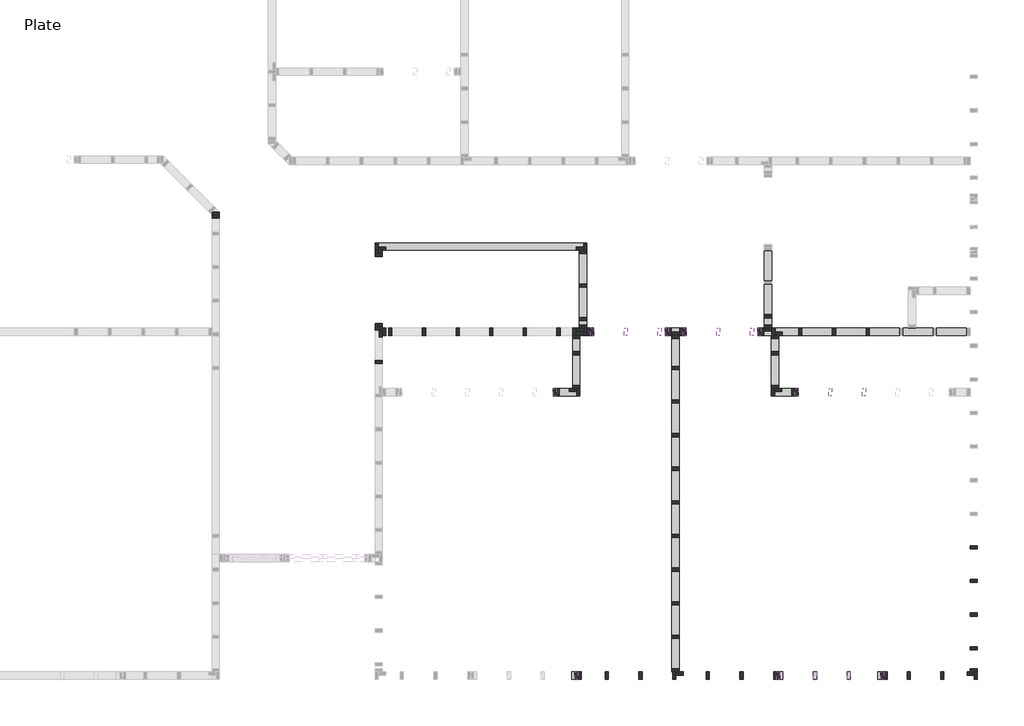
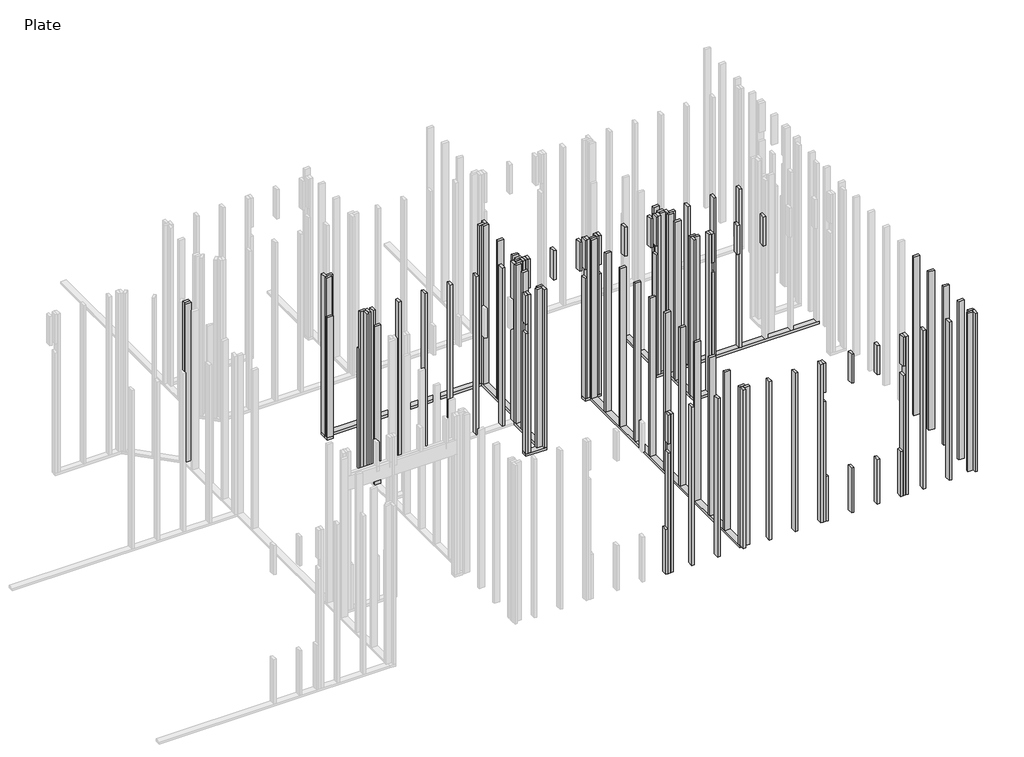
# One storey, part 2 of 5: 112 columns, 11 beams.
"""IFC4 building model written with IfcOpenShell, lengths in millimetres."""

import ifcopenshell
import ifcopenshell.guid

model = None  # the IFC model being written
_history = None  # IfcOwnerHistory: only IFC2X3 demands one
_inside = {}  # id of a spatial element -> (the spatial element, [elements in it])
_under = {}  # id of a project, library or spatial element -> (it, [spatial elements below it])
_declared = {}  # id of a project -> (the project, [libraries it declares])
_typed = {}  # id of a type object -> (the type object, [elements of that type])
_made_of = {}  # id of a material, layer set ... -> (it, [elements and type objects made of it])


def new_model(schema):
    """Start an empty IFC model of exactly this schema.

    Asked for "IFC4X3", IfcOpenShell would pick the latest addendum, in which some entities
    have other attributes; the version numbers below select the first issue.
    IFC2X3 requires an IfcOwnerHistory on every rooted entity: one is made here for all.
    """
    global model, _history
    if schema == "IFC4X3":
        model = ifcopenshell.file(schema_version=(4, 3, 0, 0))
    else:
        model = ifcopenshell.file(schema=schema)
    _inside.clear()
    _under.clear()
    _declared.clear()
    _typed.clear()
    _made_of.clear()
    _history = None
    if model.schema == "IFC2X3":
        org = make("IfcOrganization", Name="unknown")
        user = make(
            "IfcPersonAndOrganization",
            ThePerson=make("IfcPerson", FamilyName="unknown"),
            TheOrganization=org,
        )
        app = make(
            "IfcApplication",
            ApplicationDeveloper=org,
            Version="unknown",
            ApplicationFullName="unknown",
            ApplicationIdentifier="unknown",
        )
        _history = make(
            "IfcOwnerHistory",
            OwningUser=user,
            OwningApplication=app,
            ChangeAction="ADDED",
            CreationDate=0,
        )
    return model


def make(cls, **values):
    """One entity of the class cls with the attributes given. An attribute that is None is left unset."""
    return model.create_entity(
        cls, **{name: value for name, value in values.items() if value is not None}
    )


def rooted(cls, **values):
    """An entity with a GlobalId (a new one), such as an element, a storey or a relation."""
    return make(cls, GlobalId=ifcopenshell.guid.new(), OwnerHistory=_history, **values)


def si_unit(unit_type, name, prefix=None):
    """IfcSIUnit, for example si_unit("LENGTHUNIT", "METRE", prefix="MILLI")."""
    return make("IfcSIUnit", UnitType=unit_type, Prefix=prefix, Name=name)


def assignment(units):
    """IfcUnitAssignment: the units of a project."""
    return None if units is None else make("IfcUnitAssignment", Units=units)


def point(xyz):
    """IfcCartesianPoint."""
    return None if xyz is None else make("IfcCartesianPoint", Coordinates=xyz)


def direction(xyz):
    """IfcDirection."""
    return None if xyz is None else make("IfcDirection", DirectionRatios=xyz)


def frame(location, z_axis=None, x_axis=None):
    """IfcAxis2Placement3D, a coordinate frame: its origin and axes. An axis left out is left unset."""
    return make(
        "IfcAxis2Placement3D",
        Location=point(location),
        Axis=direction(z_axis),
        RefDirection=direction(x_axis),
    )


def origin():
    """The frame at (0, 0, 0) with its axes left unset."""
    return frame((0.0, 0.0, 0.0))


def place(relative_to, where):
    """IfcLocalPlacement: puts the frame where relative to a parent placement (None: the world)."""
    return make(
        "IfcLocalPlacement", PlacementRelTo=relative_to, RelativePlacement=where
    )


def context(
    kind, dimensions, precision=None, world=None, true_north=None, identifier=None
):
    """IfcGeometricRepresentationContext, for example the 3D "Model" context."""
    return make(
        "IfcGeometricRepresentationContext",
        ContextIdentifier=identifier,
        ContextType=kind,
        CoordinateSpaceDimension=dimensions,
        Precision=precision,
        WorldCoordinateSystem=world,
        TrueNorth=true_north,
    )


def project(units=None, contexts=None):
    """IfcProject with its units and contexts."""
    return rooted(
        "IfcProject",
        Name="project",
        RepresentationContexts=contexts,
        UnitsInContext=assignment(units),
    )


def spatial(cls, under=None, at=None, **own):
    """A site, building, storey or space (cls), placed at a placement, below another one or the project."""
    s = rooted(cls, ObjectPlacement=at, **own)
    if under is not None:
        _under.setdefault(under.id(), (under, []))[1].append(s)
    return s


def polyline(points):
    """IfcPolyline through the points."""
    return make("IfcPolyline", Points=[point(p) for p in points])


def outline(outer, holes=None, kind="AREA"):
    """IfcArbitraryClosedProfileDef: a profile drawn as a closed curve; with holes, ...WithVoids."""
    if holes is None:
        return make("IfcArbitraryClosedProfileDef", ProfileType=kind, OuterCurve=outer)
    return make(
        "IfcArbitraryProfileDefWithVoids",
        ProfileType=kind,
        OuterCurve=outer,
        InnerCurves=holes,
    )


def extrude(swept, where, along, depth):
    """IfcExtrudedAreaSolid: the profile swept, set in the frame where, extruded along a direction by depth."""
    return make(
        "IfcExtrudedAreaSolid",
        SweptArea=swept,
        Position=where,
        ExtrudedDirection=direction(along),
        Depth=depth,
    )


def shape(context_of_items, identifier, shape_type, items):
    """IfcShapeRepresentation: the items that make up one representation, for example the "Body"."""
    return make(
        "IfcShapeRepresentation",
        ContextOfItems=context_of_items,
        RepresentationIdentifier=identifier,
        RepresentationType=shape_type,
        Items=items,
    )


def source(mapping_origin, context_of_items, identifier, shape_type, items):
    """IfcRepresentationMap: a shape defined once, which mapped items show again and again."""
    return make(
        "IfcRepresentationMap",
        MappingOrigin=mapping_origin,
        MappedRepresentation=shape(context_of_items, identifier, shape_type, items),
    )


def transform(
    local_origin,
    x_axis=None,
    y_axis=None,
    z_axis=None,
    scale=None,
    scale2=None,
    scale3=None,
    uniform=True,
):
    """IfcCartesianTransformationOperator3D, or its non-uniform kind. x_axis, y_axis, z_axis: its Axis1, 2, 3."""
    if uniform:
        return make(
            "IfcCartesianTransformationOperator3D",
            Axis1=direction(x_axis),
            Axis2=direction(y_axis),
            LocalOrigin=point(local_origin),
            Scale=scale,
            Axis3=direction(z_axis),
        )
    return make(
        "IfcCartesianTransformationOperator3DnonUniform",
        Axis1=direction(x_axis),
        Axis2=direction(y_axis),
        LocalOrigin=point(local_origin),
        Scale=scale,
        Axis3=direction(z_axis),
        Scale2=scale2,
        Scale3=scale3,
    )


def mapped(mapping_source, mapping_target):
    """IfcMappedItem: shows the shape of a source again, moved by a transform."""
    return make(
        "IfcMappedItem", MappingSource=mapping_source, MappingTarget=mapping_target
    )


def made_of(thing, what):
    """Note that an element or type object is made of a material, layer set ...; save() writes the relation."""
    if what is not None:
        _made_of.setdefault(what.id(), (what, []))[1].append(thing)
    return thing


def element(
    cls,
    number,
    at=None,
    inside=None,
    cuts=None,
    type_object=None,
    material=None,
    context=None,
    identifier="Body",
    shape_type=None,
    held_by="IfcProductDefinitionShape",
    body=None,
    shapes=None,
    **own,
):
    """One element of the class cls, such as IfcWall. Its Tag is "e" and its number.

    at: its placement. inside: the storey or other place that contains it. cuts: it is an
    opening in that element (IfcRelVoidsElement). A single representation is given by context,
    identifier, shape_type and body (its items); several are given by shapes. held_by: the class
    of the entity that holds the representations. save() writes the other relations.
    """
    e = rooted(cls, Tag="e%d" % number, ObjectPlacement=at, **own)
    if body is not None:
        shapes = [shape(context, identifier, shape_type, body)]
    if shapes is not None:
        e.Representation = make(held_by, Representations=shapes)
    if inside is not None:
        _inside.setdefault(inside.id(), (inside, []))[1].append(e)
    if cuts is not None:
        rooted(
            "IfcRelVoidsElement", RelatingBuildingElement=cuts, RelatedOpeningElement=e
        )
    if type_object is not None:
        _typed.setdefault(type_object.id(), (type_object, []))[1].append(e)
    return made_of(e, material)


def aggregate(whole, parts):
    """IfcRelAggregates: a whole, such as a stair, and the parts it consists of."""
    return rooted("IfcRelAggregates", RelatingObject=whole, RelatedObjects=parts)


def save(model, path):
    """Write the relations noted so far, then the file.

    IfcRelAggregates (storeys below a building ...), IfcRelContainedInSpatialStructure (elements
    in a storey), IfcRelDefinesByType, IfcRelAssociatesMaterial and IfcRelDeclares: one each for
    every whole, place, type object, material and project.
    """
    for whole, parts in _under.values():
        aggregate(whole, parts)
    for where, things in _inside.values():
        rooted(
            "IfcRelContainedInSpatialStructure",
            RelatedElements=things,
            RelatingStructure=where,
        )
    for kind, things in _typed.values():
        rooted("IfcRelDefinesByType", RelatedObjects=things, RelatingType=kind)
    for what, things in _made_of.values():
        rooted("IfcRelAssociatesMaterial", RelatedObjects=things, RelatingMaterial=what)
    for by, libraries in _declared.values():
        rooted("IfcRelDeclares", RelatingContext=by, RelatedDefinitions=libraries)
    model.write(path)


def dimension_lumber_supporting_bottom_plate_c90501c4(model_context):
    return source(origin(), model_context, "Body", "SweptSolid", [
        extrude(outline(polyline([(1306.3140625, 44.45), (1306.3140625, -44.45), (-1261.8640625, -44.45), (-1261.8640625, 44.45), (1306.3140625, 44.45)])), frame((0.0, 0.0, -19.05), z_axis=(0.0, 0.0, 1.0), x_axis=(1.0, 0.0, 0.0)), (0.0, 0.0, 1.0), 38.1),
    ])


def dimension_lumber_supporting_bottom_plate_879a6a2b(model_context):
    return source(origin(), model_context, "Body", "SweptSolid", [
        extrude(outline(polyline([(2009.775, 44.45), (2009.775, -44.45), (-2060.575, -44.45), (-2060.575, 44.45), (2009.775, 44.45)])), frame((0.0, 0.0, -19.05), z_axis=(0.0, 0.0, 1.0), x_axis=(1.0, 0.0, 0.0)), (0.0, 0.0, 1.0), 38.1),
    ])


def dimension_lumber_supporting_bottom_plate_90e85d83(model_context):
    return source(origin(), model_context, "Body", "SweptSolid", [
        extrude(outline(polyline([(128.190625, 44.45), (128.190625, -44.45), (-128.190625, -44.45), (-128.190625, 44.45), (128.190625, 44.45)])), frame((0.0, 0.0, -19.05), z_axis=(0.0, 0.0, 1.0), x_axis=(1.0, 0.0, 0.0)), (0.0, 0.0, 1.0), 38.1),
    ])


def dimension_lumber_supporting_bottom_plate_7dbe58bc(model_context):
    return source(origin(), model_context, "Body", "SweptSolid", [
        extrude(outline(polyline([(469.9, 44.45), (469.9, -44.45), (-469.9, -44.45), (-469.9, 44.45), (469.9, 44.45)])), frame((0.0, 0.0, -19.05), z_axis=(0.0, 0.0, 1.0), x_axis=(1.0, 0.0, 0.0)), (0.0, 0.0, 1.0), 38.1),
    ])


def dimension_lumber_supporting_bottom_plate_050ef5e1(model_context):
    return source(origin(), model_context, "Body", "SweptSolid", [
        extrude(outline(polyline([(1279.525, 44.45), (1279.525, -44.45), (-1279.525, -44.45), (-1279.525, 44.45), (1279.525, 44.45)])), frame((0.0, 0.0, -19.05), z_axis=(0.0, 0.0, 1.0), x_axis=(1.0, 0.0, 0.0)), (0.0, 0.0, 1.0), 38.1),
    ])


def dimension_lumber_supporting_bottom_plate_723ed126(model_context):
    return source(origin(), model_context, "Body", "SweptSolid", [
        extrude(outline(polyline([(60.325, 44.45), (60.325, -44.45), (-15.875, -44.45), (-15.875, 44.45), (60.325, 44.45)])), frame((0.0, 0.0, -19.05), z_axis=(0.0, 0.0, 1.0), x_axis=(1.0, 0.0, 0.0)), (0.0, 0.0, 1.0), 38.1),
    ])


def dimension_lumber_supporting_bottom_plate_fcdf3739(model_context):
    return source(origin(), model_context, "Body", "SweptSolid", [
        extrude(outline(polyline([(352.425, 44.45), (352.425, -44.45), (-288.925, -44.45), (-288.925, 44.45), (352.425, 44.45)])), frame((0.0, 0.0, -19.05), z_axis=(0.0, 0.0, 1.0), x_axis=(1.0, 0.0, 0.0)), (0.0, 0.0, 1.0), 38.1),
    ])


def dimension_lumber_supporting_bottom_plate_c78b9630(model_context):
    return source(origin(), model_context, "Body", "SweptSolid", [
        extrude(outline(polyline([(488.95, 44.45), (488.95, -44.45), (-521.890625, -44.45), (-521.890625, 44.45), (488.95, 44.45)])), frame((0.0, 0.0, -19.05), z_axis=(0.0, 0.0, 1.0), x_axis=(1.0, 0.0, 0.0)), (0.0, 0.0, 1.0), 38.1),
    ])


def dimension_lumber_supporting_bottom_plate_50cface6(model_context):
    return source(origin(), model_context, "Body", "SweptSolid", [
        extrude(outline(polyline([(320.675, 44.45), (320.675, -44.45), (-320.675, -44.45), (-320.675, 44.45), (320.675, 44.45)])), frame((0.0, 0.0, -19.05), z_axis=(0.0, 0.0, 1.0), x_axis=(1.0, 0.0, 0.0)), (0.0, 0.0, 1.0), 38.1),
    ])


def dimension_lumber_supporting_bottom_plate_f7639587(model_context):
    return source(origin(), model_context, "Body", "SweptSolid", [
        extrude(outline(polyline([(184.9437503, 44.45), (184.9437503, -44.45), (-140.4937503, -44.45), (-140.4937503, 44.45), (184.9437503, 44.45)])), frame((0.0, 0.0, -19.05), z_axis=(0.0, 0.0, 1.0), x_axis=(1.0, 0.0, 0.0)), (0.0, 0.0, 1.0), 38.1),
    ])


def dimension_lumber_supporting_bottom_plate_f386abe9(model_context):
    return source(origin(), model_context, "Body", "SweptSolid", [
        extrude(outline(polyline([(184.15, 44.45), (184.15, -44.45), (-139.7, -44.45), (-139.7, 44.45), (184.15, 44.45)])), frame((0.0, 0.0, -19.05), z_axis=(0.0, 0.0, 1.0), x_axis=(1.0, 0.0, 0.0)), (0.0, 0.0, 1.0), 38.1),
    ])


def dimension_lumber_column_2x4_07183c39(model_context):
    return source(origin(), model_context, "Body", "SweptSolid", [
        extrude(outline(polyline([(19.05, 44.45), (19.05, -44.45), (-19.05, -44.45), (-19.05, 44.45), (19.05, 44.45)])), frame((0.0, 0.0, 56.35625), z_axis=(0.0, 0.0, 1.0), x_axis=(1.0, 0.0, 0.0)), (0.0, 0.0, 1.0), 2636.04375),
    ])


def dimension_lumber_column_2x4_f24b5bbb(model_context):
    return source(origin(), model_context, "Body", "SweptSolid", [
        extrude(outline(polyline([(19.05, -44.45), (-19.05, -44.45), (-19.05, 44.45), (19.05, 44.45), (19.05, -44.45)])), frame((0.0, 0.0, 56.35625), z_axis=(0.0, 0.0, 1.0), x_axis=(1.0, 0.0, 0.0)), (0.0, 0.0, 1.0), 2636.04375),
    ])


def dimension_lumber_column_2x4_0f816ddf(model_context):
    return source(origin(), model_context, "Body", "SweptSolid", [
        extrude(outline(polyline([(19.05, 44.45), (19.05, -44.45), (-19.05, -44.45), (-19.05, 44.45), (19.05, 44.45)])), frame((0.0, 0.0, 56.35625), z_axis=(0.0, 0.0, 1.0), x_axis=(1.0, 0.0, 0.0)), (0.0, 0.0, 1.0), 1999.853125),
    ])


def dimension_lumber_column_2x4_c2f848da(model_context):
    return source(origin(), model_context, "Body", "SweptSolid", [
        extrude(outline(polyline([(19.05, 44.45), (19.05, -44.45), (-19.05, -44.45), (-19.05, 44.45), (19.05, 44.45)])), frame((0.0, 0.0, 2208.609375), z_axis=(0.0, 0.0, 1.0), x_axis=(1.0, 0.0, 0.0)), (0.0, 0.0, 1.0), 483.790625),
    ])


def dimension_lumber_column_2x4_35883525(model_context):
    return source(origin(), model_context, "Body", "SweptSolid", [
        extrude(outline(polyline([(19.05, 44.45), (19.05, -44.45), (-19.05, -44.45), (-19.05, 44.45), (19.05, 44.45)])), frame((0.0, 0.0, 56.35625), z_axis=(0.0, 0.0, 1.0), x_axis=(1.0, 0.0, 0.0)), (0.0, 0.0, 1.0), 742.553125),
    ])


model = new_model("IFC4")

# Units and contexts
model_context = context("Model", 3, world=origin())
ifc_project = project(units=[si_unit("LENGTHUNIT", "METRE", prefix="MILLI")], contexts=[model_context])

# Site, building, storey
site = spatial("IfcSite", under=ifc_project)
building = spatial("IfcBuilding", under=site)
storey = spatial("IfcBuildingStorey", under=building, Name="Plate", Elevation=56.35625)

# Beams
placement = place(None, origin())
dimension_lumber_supporting_bottom_plate_shape = dimension_lumber_supporting_bottom_plate_c90501c4(model_context)
element("IfcBeam", 1, ObjectType="Dimension Lumber : Supporting Bottom Plate", at=placement, inside=storey, context=model_context, shape_type="MappedRepresentation", body=[
    mapped(dimension_lumber_supporting_bottom_plate_shape, transform((11893.3082124, -1545.8540947, 37.30625), x_axis=(-1.0, 0.0, 0.0), y_axis=(0.0, -1.0, 0.0), z_axis=(0.0, 0.0, 1.0))),
])
dimension_lumber_supporting_bottom_plate_2_shape = dimension_lumber_supporting_bottom_plate_879a6a2b(model_context)
element("IfcBeam", 2, ObjectType="Dimension Lumber : Supporting Bottom Plate", at=placement, inside=storey, context=model_context, shape_type="MappedRepresentation", body=[
    mapped(dimension_lumber_supporting_bottom_plate_2_shape, transform((9597.5847749, -3600.0790947, 37.30625), x_axis=(0.0, 1.0, 0.0), y_axis=(-1.0, 0.0, 0.0), z_axis=(0.0, 0.0, 1.0))),
])
dimension_lumber_supporting_bottom_plate_3_shape = dimension_lumber_supporting_bottom_plate_90e85d83(model_context)
element("IfcBeam", 3, ObjectType="Dimension Lumber : Supporting Bottom Plate", at=placement, inside=storey, context=model_context, shape_type="MappedRepresentation", body=[
    mapped(dimension_lumber_supporting_bottom_plate_3_shape, transform((9597.5847749, -1545.8540947, 37.30625), x_axis=(-1.0, 0.0, 0.0), y_axis=(0.0, -1.0, 0.0), z_axis=(0.0, 0.0, 1.0))),
])
dimension_lumber_supporting_bottom_plate_4_shape = dimension_lumber_supporting_bottom_plate_7dbe58bc(model_context)
element("IfcBeam", 4, ObjectType="Dimension Lumber : Supporting Bottom Plate", at=placement, inside=storey, context=model_context, shape_type="MappedRepresentation", body=[
    mapped(dimension_lumber_supporting_bottom_plate_4_shape, transform((8479.9847749, -1031.5040947, 37.30625), x_axis=(0.0, 1.0, 0.0), y_axis=(-1.0, 0.0, 0.0), z_axis=(0.0, 0.0, 1.0))),
])
dimension_lumber_supporting_bottom_plate_5_shape = dimension_lumber_supporting_bottom_plate_050ef5e1(model_context)
element("IfcBeam", 5, ObjectType="Dimension Lumber : Supporting Bottom Plate", at=placement, inside=storey, context=model_context, shape_type="MappedRepresentation", body=[
    mapped(dimension_lumber_supporting_bottom_plate_5_shape, transform((7244.9097749, -517.1540947, 37.30625), x_axis=(-1.0, 0.0, 0.0), y_axis=(0.0, -1.0, 0.0), z_axis=(0.0, 0.0, 1.0))),
])
dimension_lumber_supporting_bottom_plate_6_shape = dimension_lumber_supporting_bottom_plate_723ed126(model_context)
element("IfcBeam", 6, ObjectType="Dimension Lumber : Supporting Bottom Plate", at=placement, inside=storey, context=model_context, shape_type="MappedRepresentation", body=[
    mapped(dimension_lumber_supporting_bottom_plate_6_shape, transform((6009.8347749, -577.4790947, 37.30625), x_axis=(0.0, -1.0, 0.0), y_axis=(1.0, 0.0, 0.0), z_axis=(0.0, 0.0, 1.0))),
])
dimension_lumber_supporting_bottom_plate_7_shape = dimension_lumber_supporting_bottom_plate_fcdf3739(model_context)
element("IfcBeam", 7, ObjectType="Dimension Lumber : Supporting Bottom Plate", at=placement, inside=storey, context=model_context, shape_type="MappedRepresentation", body=[
    mapped(dimension_lumber_supporting_bottom_plate_7_shape, transform((8397.4347755, -1942.7290947, 37.30625), x_axis=(0.0, 1.0, 0.0), y_axis=(-1.0, 0.0, 0.0), z_axis=(0.0, 0.0, 1.0))),
])
dimension_lumber_supporting_bottom_plate_8_shape = dimension_lumber_supporting_bottom_plate_c78b9630(model_context)
element("IfcBeam", 8, ObjectType="Dimension Lumber : Supporting Bottom Plate", at=placement, inside=storey, context=model_context, shape_type="MappedRepresentation", body=[
    mapped(dimension_lumber_supporting_bottom_plate_8_shape, transform((10715.1847749, -1012.4540947, 37.30625), x_axis=(0.0, -1.0, 0.0), y_axis=(1.0, 0.0, 0.0), z_axis=(0.0, 0.0, 1.0))),
])
dimension_lumber_supporting_bottom_plate_9_shape = dimension_lumber_supporting_bottom_plate_50cface6(model_context)
element("IfcBeam", 9, ObjectType="Dimension Lumber : Supporting Bottom Plate", at=placement, inside=storey, context=model_context, shape_type="MappedRepresentation", body=[
    mapped(dimension_lumber_supporting_bottom_plate_9_shape, transform((10799.3222749, -1910.9790947, 37.30625), x_axis=(0.0, 1.0, 0.0), y_axis=(-1.0, 0.0, 0.0), z_axis=(0.0, 0.0, 1.0))),
])
dimension_lumber_supporting_bottom_plate_10_shape = dimension_lumber_supporting_bottom_plate_f7639587(model_context)
element("IfcBeam", 10, ObjectType="Dimension Lumber : Supporting Bottom Plate", at=placement, inside=storey, context=model_context, shape_type="MappedRepresentation", body=[
    mapped(dimension_lumber_supporting_bottom_plate_10_shape, transform((8256.9410252, -2276.1040947, 37.30625), x_axis=(1.0, 0.0, 0.0), y_axis=(0.0, 1.0, 0.0), z_axis=(0.0, 0.0, 1.0))),
])
dimension_lumber_supporting_bottom_plate_11_shape = dimension_lumber_supporting_bottom_plate_f386abe9(model_context)
element("IfcBeam", 11, ObjectType="Dimension Lumber : Supporting Bottom Plate", at=placement, inside=storey, context=model_context, shape_type="MappedRepresentation", body=[
    mapped(dimension_lumber_supporting_bottom_plate_11_shape, transform((10939.0222749, -2276.1040947, 37.30625), x_axis=(-1.0, 0.0, 0.0), y_axis=(0.0, -1.0, 0.0), z_axis=(0.0, 0.0, 1.0))),
])

# Columns
dimension_lumber_column_2x4_shape = dimension_lumber_column_2x4_07183c39(model_context)
element("IfcColumn", 12, ObjectType="Dimension Lumber-Column : 2x4", at=placement, inside=storey, context=model_context, shape_type="MappedRepresentation", body=[
    mapped(dimension_lumber_column_2x4_shape, transform((10799.3222749, -5705.1040947, 0.0), x_axis=(1.0, 0.0, 0.0), y_axis=(0.0, 1.0, 0.0), z_axis=(0.0, 0.0, 1.0))),
])
element("IfcColumn", 13, ObjectType="Dimension Lumber-Column : 2x4", at=placement, inside=storey, context=model_context, shape_type="MappedRepresentation", body=[
    mapped(dimension_lumber_column_2x4_shape, transform((10392.9222749, -5705.1040947, 0.0), x_axis=(1.0, 0.0, 0.0), y_axis=(0.0, 1.0, 0.0), z_axis=(0.0, 0.0, 1.0))),
])
element("IfcColumn", 14, ObjectType="Dimension Lumber-Column : 2x4", at=placement, inside=storey, context=model_context, shape_type="MappedRepresentation", body=[
    mapped(dimension_lumber_column_2x4_shape, transform((9986.5222749, -5705.1040947, 0.0), x_axis=(1.0, 0.0, 0.0), y_axis=(0.0, 1.0, 0.0), z_axis=(0.0, 0.0, 1.0))),
])
element("IfcColumn", 15, ObjectType="Dimension Lumber-Column : 2x4", at=placement, inside=storey, context=model_context, shape_type="MappedRepresentation", body=[
    mapped(dimension_lumber_column_2x4_shape, transform((9580.1222749, -5705.1040947, 0.0), x_axis=(1.0, 0.0, 0.0), y_axis=(0.0, 1.0, 0.0), z_axis=(0.0, 0.0, 1.0))),
])
element("IfcColumn", 16, ObjectType="Dimension Lumber-Column : 2x4", at=placement, inside=storey, context=model_context, shape_type="MappedRepresentation", body=[
    mapped(dimension_lumber_column_2x4_shape, transform((9173.7222749, -5705.1040947, 0.0), x_axis=(1.0, 0.0, 0.0), y_axis=(0.0, 1.0, 0.0), z_axis=(0.0, 0.0, 1.0))),
])
element("IfcColumn", 17, ObjectType="Dimension Lumber-Column : 2x4", at=placement, inside=storey, context=model_context, shape_type="MappedRepresentation", body=[
    mapped(dimension_lumber_column_2x4_shape, transform((8767.3222749, -5705.1040947, 0.0), x_axis=(1.0, 0.0, 0.0), y_axis=(0.0, 1.0, 0.0), z_axis=(0.0, 0.0, 1.0))),
])
element("IfcColumn", 18, ObjectType="Dimension Lumber-Column : 2x4", at=placement, inside=storey, context=model_context, shape_type="MappedRepresentation", body=[
    mapped(dimension_lumber_column_2x4_shape, transform((13199.6222749, -4154.1165947, 0.0), x_axis=(0.0, 1.0, 0.0), y_axis=(-1.0, 0.0, 0.0), z_axis=(0.0, 0.0, 1.0))),
])
element("IfcColumn", 19, ObjectType="Dimension Lumber-Column : 2x4", at=placement, inside=storey, context=model_context, shape_type="MappedRepresentation", body=[
    mapped(dimension_lumber_column_2x4_shape, transform((13199.6222749, -4560.5165947, 0.0), x_axis=(0.0, 1.0, 0.0), y_axis=(-1.0, 0.0, 0.0), z_axis=(0.0, 0.0, 1.0))),
])
element("IfcColumn", 20, ObjectType="Dimension Lumber-Column : 2x4", at=placement, inside=storey, context=model_context, shape_type="MappedRepresentation", body=[
    mapped(dimension_lumber_column_2x4_shape, transform((13199.6222749, -4966.9165947, 0.0), x_axis=(0.0, 1.0, 0.0), y_axis=(-1.0, 0.0, 0.0), z_axis=(0.0, 0.0, 1.0))),
])
element("IfcColumn", 21, ObjectType="Dimension Lumber-Column : 2x4", at=placement, inside=storey, context=model_context, shape_type="MappedRepresentation", body=[
    mapped(dimension_lumber_column_2x4_shape, transform((13199.6222749, -5373.3165947, 0.0), x_axis=(0.0, 1.0, 0.0), y_axis=(-1.0, 0.0, 0.0), z_axis=(0.0, 0.0, 1.0))),
])
element("IfcColumn", 22, ObjectType="Dimension Lumber-Column : 2x4", at=placement, inside=storey, context=model_context, shape_type="MappedRepresentation", body=[
    mapped(dimension_lumber_column_2x4_shape, transform((11916.9222749, -1545.8540947, 0.0), x_axis=(1.0, 0.0, 0.0), y_axis=(0.0, 1.0, 0.0), z_axis=(0.0, 0.0, 1.0))),
])
element("IfcColumn", 23, ObjectType="Dimension Lumber-Column : 2x4", at=placement, inside=storey, context=model_context, shape_type="MappedRepresentation", body=[
    mapped(dimension_lumber_column_2x4_shape, transform((11510.5222749, -1545.8540947, 0.0), x_axis=(1.0, 0.0, 0.0), y_axis=(0.0, 1.0, 0.0), z_axis=(0.0, 0.0, 1.0))),
])
element("IfcColumn", 24, ObjectType="Dimension Lumber-Column : 2x4", at=placement, inside=storey, context=model_context, shape_type="MappedRepresentation", body=[
    mapped(dimension_lumber_column_2x4_shape, transform((11104.1222749, -1545.8540947, 0.0), x_axis=(1.0, 0.0, 0.0), y_axis=(0.0, 1.0, 0.0), z_axis=(0.0, 0.0, 1.0))),
])
element("IfcColumn", 25, ObjectType="Dimension Lumber-Column : 2x4", at=placement, inside=storey, context=model_context, shape_type="MappedRepresentation", body=[
    mapped(dimension_lumber_column_2x4_shape, transform((10780.2722749, -1545.8540947, 0.0), x_axis=(1.0, 0.0, 0.0), y_axis=(0.0, 1.0, 0.0), z_axis=(0.0, 0.0, 1.0))),
])
element("IfcColumn", 26, ObjectType="Dimension Lumber-Column : 2x4", at=placement, inside=storey, context=model_context, shape_type="MappedRepresentation", body=[
    mapped(dimension_lumber_column_2x4_shape, transform((8182.7253999, -1545.8540947, 0.0), x_axis=(1.0, 0.0, 0.0), y_axis=(0.0, 1.0, 0.0), z_axis=(0.0, 0.0, 1.0))),
])
element("IfcColumn", 27, ObjectType="Dimension Lumber-Column : 2x4", at=placement, inside=storey, context=model_context, shape_type="MappedRepresentation", body=[
    mapped(dimension_lumber_column_2x4_shape, transform((7776.3253999, -1545.8540947, 0.0), x_axis=(1.0, 0.0, 0.0), y_axis=(0.0, 1.0, 0.0), z_axis=(0.0, 0.0, 1.0))),
])
element("IfcColumn", 28, ObjectType="Dimension Lumber-Column : 2x4", at=placement, inside=storey, context=model_context, shape_type="MappedRepresentation", body=[
    mapped(dimension_lumber_column_2x4_shape, transform((7369.9253999, -1545.8540947, 0.0), x_axis=(1.0, 0.0, 0.0), y_axis=(0.0, 1.0, 0.0), z_axis=(0.0, 0.0, 1.0))),
])
element("IfcColumn", 29, ObjectType="Dimension Lumber-Column : 2x4", at=placement, inside=storey, context=model_context, shape_type="MappedRepresentation", body=[
    mapped(dimension_lumber_column_2x4_shape, transform((6963.5253999, -1545.8540947, 0.0), x_axis=(1.0, 0.0, 0.0), y_axis=(0.0, 1.0, 0.0), z_axis=(0.0, 0.0, 1.0))),
])
element("IfcColumn", 30, ObjectType="Dimension Lumber-Column : 2x4", at=placement, inside=storey, context=model_context, shape_type="MappedRepresentation", body=[
    mapped(dimension_lumber_column_2x4_shape, transform((6557.1253999, -1545.8540947, 0.0), x_axis=(1.0, 0.0, 0.0), y_axis=(0.0, 1.0, 0.0), z_axis=(0.0, 0.0, 1.0))),
])
element("IfcColumn", 31, ObjectType="Dimension Lumber-Column : 2x4", at=placement, inside=storey, context=model_context, shape_type="MappedRepresentation", body=[
    mapped(dimension_lumber_column_2x4_shape, transform((6150.7253999, -1545.8540947, 0.0), x_axis=(1.0, 0.0, 0.0), y_axis=(0.0, 1.0, 0.0), z_axis=(0.0, 0.0, 1.0))),
])
element("IfcColumn", 32, ObjectType="Dimension Lumber-Column : 2x4", at=placement, inside=storey, context=model_context, shape_type="MappedRepresentation", body=[
    mapped(dimension_lumber_column_2x4_shape, transform((9668.6253999, -1545.8540947, 0.0), x_axis=(1.0, 0.0, 0.0), y_axis=(0.0, 1.0, 0.0), z_axis=(0.0, 0.0, 1.0))),
])
element("IfcColumn", 33, ObjectType="Dimension Lumber-Column : 2x4", at=placement, inside=storey, context=model_context, shape_type="MappedRepresentation", body=[
    mapped(dimension_lumber_column_2x4_shape, transform((8551.0253999, -1545.8540947, 0.0), x_axis=(1.0, 0.0, 0.0), y_axis=(0.0, 1.0, 0.0), z_axis=(0.0, 0.0, 1.0))),
])
element("IfcColumn", 34, ObjectType="Dimension Lumber-Column : 2x4", at=placement, inside=storey, context=model_context, shape_type="MappedRepresentation", body=[
    mapped(dimension_lumber_column_2x4_shape, transform((9526.5441499, -1545.8540947, 0.0), x_axis=(1.0, 0.0, 0.0), y_axis=(0.0, 1.0, 0.0), z_axis=(0.0, 0.0, 1.0))),
])
element("IfcColumn", 35, ObjectType="Dimension Lumber-Column : 2x4", at=placement, inside=storey, context=model_context, shape_type="MappedRepresentation", body=[
    mapped(dimension_lumber_column_2x4_shape, transform((10644.1441499, -1545.8540947, 0.0), x_axis=(1.0, 0.0, 0.0), y_axis=(0.0, 1.0, 0.0), z_axis=(0.0, 0.0, 1.0))),
])
element("IfcColumn", 36, ObjectType="Dimension Lumber-Column : 2x4", at=placement, inside=storey, context=model_context, shape_type="MappedRepresentation", body=[
    mapped(dimension_lumber_column_2x4_shape, transform((9597.5847749, -5641.6040947, 0.0), x_axis=(0.0, 1.0, 0.0), y_axis=(-1.0, 0.0, 0.0), z_axis=(0.0, 0.0, 1.0))),
])
element("IfcColumn", 37, ObjectType="Dimension Lumber-Column : 2x4", at=placement, inside=storey, context=model_context, shape_type="MappedRepresentation", body=[
    mapped(dimension_lumber_column_2x4_shape, transform((9643.6222749, -5679.7040947, 0.0), x_axis=(0.0, 1.0, 0.0), y_axis=(-1.0, 0.0, 0.0), z_axis=(0.0, 0.0, 1.0))),
])
element("IfcColumn", 38, ObjectType="Dimension Lumber-Column : 2x4", at=placement, inside=storey, context=model_context, shape_type="MappedRepresentation", body=[
    mapped(dimension_lumber_column_2x4_shape, transform((9597.5847749, -5235.2040947, 0.0), x_axis=(0.0, 1.0, 0.0), y_axis=(-1.0, 0.0, 0.0), z_axis=(0.0, 0.0, 1.0))),
])
element("IfcColumn", 39, ObjectType="Dimension Lumber-Column : 2x4", at=placement, inside=storey, context=model_context, shape_type="MappedRepresentation", body=[
    mapped(dimension_lumber_column_2x4_shape, transform((9597.5847749, -4828.8040947, 0.0), x_axis=(0.0, 1.0, 0.0), y_axis=(-1.0, 0.0, 0.0), z_axis=(0.0, 0.0, 1.0))),
])
element("IfcColumn", 40, ObjectType="Dimension Lumber-Column : 2x4", at=placement, inside=storey, context=model_context, shape_type="MappedRepresentation", body=[
    mapped(dimension_lumber_column_2x4_shape, transform((9597.5847749, -4422.4040947, 0.0), x_axis=(0.0, 1.0, 0.0), y_axis=(-1.0, 0.0, 0.0), z_axis=(0.0, 0.0, 1.0))),
])
element("IfcColumn", 41, ObjectType="Dimension Lumber-Column : 2x4", at=placement, inside=storey, context=model_context, shape_type="MappedRepresentation", body=[
    mapped(dimension_lumber_column_2x4_shape, transform((9597.5847749, -4016.0040947, 0.0), x_axis=(0.0, 1.0, 0.0), y_axis=(-1.0, 0.0, 0.0), z_axis=(0.0, 0.0, 1.0))),
])
element("IfcColumn", 42, ObjectType="Dimension Lumber-Column : 2x4", at=placement, inside=storey, context=model_context, shape_type="MappedRepresentation", body=[
    mapped(dimension_lumber_column_2x4_shape, transform((9597.5847749, -3609.6040947, 0.0), x_axis=(0.0, 1.0, 0.0), y_axis=(-1.0, 0.0, 0.0), z_axis=(0.0, 0.0, 1.0))),
])
element("IfcColumn", 43, ObjectType="Dimension Lumber-Column : 2x4", at=placement, inside=storey, context=model_context, shape_type="MappedRepresentation", body=[
    mapped(dimension_lumber_column_2x4_shape, transform((9597.5847749, -3203.2040947, 0.0), x_axis=(0.0, 1.0, 0.0), y_axis=(-1.0, 0.0, 0.0), z_axis=(0.0, 0.0, 1.0))),
])
element("IfcColumn", 44, ObjectType="Dimension Lumber-Column : 2x4", at=placement, inside=storey, context=model_context, shape_type="MappedRepresentation", body=[
    mapped(dimension_lumber_column_2x4_shape, transform((9597.5847749, -2796.8040947, 0.0), x_axis=(0.0, 1.0, 0.0), y_axis=(-1.0, 0.0, 0.0), z_axis=(0.0, 0.0, 1.0))),
])
element("IfcColumn", 45, ObjectType="Dimension Lumber-Column : 2x4", at=placement, inside=storey, context=model_context, shape_type="MappedRepresentation", body=[
    mapped(dimension_lumber_column_2x4_shape, transform((9597.5847749, -2390.4040947, 0.0), x_axis=(0.0, 1.0, 0.0), y_axis=(-1.0, 0.0, 0.0), z_axis=(0.0, 0.0, 1.0))),
])
element("IfcColumn", 46, ObjectType="Dimension Lumber-Column : 2x4", at=placement, inside=storey, context=model_context, shape_type="MappedRepresentation", body=[
    mapped(dimension_lumber_column_2x4_shape, transform((9597.5847749, -1984.0040947, 0.0), x_axis=(0.0, 1.0, 0.0), y_axis=(-1.0, 0.0, 0.0), z_axis=(0.0, 0.0, 1.0))),
])
element("IfcColumn", 47, ObjectType="Dimension Lumber-Column : 2x4", at=placement, inside=storey, context=model_context, shape_type="MappedRepresentation", body=[
    mapped(dimension_lumber_column_2x4_shape, transform((9597.5847749, -1609.3540947, 0.0), x_axis=(0.0, 1.0, 0.0), y_axis=(-1.0, 0.0, 0.0), z_axis=(0.0, 0.0, 1.0))),
])
element("IfcColumn", 48, ObjectType="Dimension Lumber-Column : 2x4", at=placement, inside=storey, context=model_context, shape_type="MappedRepresentation", body=[
    mapped(dimension_lumber_column_2x4_shape, transform((9590.0441499, -1571.2540947, 0.0), x_axis=(0.0, 1.0, 0.0), y_axis=(-1.0, 0.0, 0.0), z_axis=(0.0, 0.0, 1.0))),
])
element("IfcColumn", 49, ObjectType="Dimension Lumber-Column : 2x4", at=placement, inside=storey, context=model_context, shape_type="MappedRepresentation", body=[
    mapped(dimension_lumber_column_2x4_shape, transform((10715.1847749, -1360.5134697, 0.0), x_axis=(0.0, 1.0, 0.0), y_axis=(-1.0, 0.0, 0.0), z_axis=(0.0, 0.0, 1.0))),
])
element("IfcColumn", 50, ObjectType="Dimension Lumber-Column : 2x4", at=placement, inside=storey, context=model_context, shape_type="MappedRepresentation", body=[
    mapped(dimension_lumber_column_2x4_shape, transform((10715.1847749, -1482.3540947, 0.0), x_axis=(0.0, 1.0, 0.0), y_axis=(-1.0, 0.0, 0.0), z_axis=(0.0, 0.0, 1.0))),
])
element("IfcColumn", 51, ObjectType="Dimension Lumber-Column : 2x4", at=placement, inside=storey, context=model_context, shape_type="MappedRepresentation", body=[
    mapped(dimension_lumber_column_2x4_shape, transform((10716.7722749, -1520.4540947, 0.0), x_axis=(0.0, 1.0, 0.0), y_axis=(-1.0, 0.0, 0.0), z_axis=(0.0, 0.0, 1.0))),
])
element("IfcColumn", 52, ObjectType="Dimension Lumber-Column : 2x4", at=placement, inside=storey, context=model_context, shape_type="MappedRepresentation", body=[
    mapped(dimension_lumber_column_2x4_shape, transform((8506.5753999, -1545.8540947, 0.0), x_axis=(1.0, 0.0, 0.0), y_axis=(0.0, 1.0, 0.0), z_axis=(0.0, 0.0, 1.0))),
])
element("IfcColumn", 53, ObjectType="Dimension Lumber-Column : 2x4", at=placement, inside=storey, context=model_context, shape_type="MappedRepresentation", body=[
    mapped(dimension_lumber_column_2x4_shape, transform((8479.9847749, -580.6540947, 0.0), x_axis=(0.0, -1.0, 0.0), y_axis=(1.0, 0.0, 0.0), z_axis=(0.0, 0.0, 1.0))),
])
element("IfcColumn", 54, ObjectType="Dimension Lumber-Column : 2x4", at=placement, inside=storey, context=model_context, shape_type="MappedRepresentation", body=[
    mapped(dimension_lumber_column_2x4_shape, transform((8441.8847749, -542.5492023, 0.0), x_axis=(0.0, -1.0, 0.0), y_axis=(1.0, 0.0, 0.0), z_axis=(0.0, 0.0, 1.0))),
])
element("IfcColumn", 55, ObjectType="Dimension Lumber-Column : 2x4", at=placement, inside=storey, context=model_context, shape_type="MappedRepresentation", body=[
    mapped(dimension_lumber_column_2x4_shape, transform((8479.9847749, -987.0540947, 0.0), x_axis=(0.0, -1.0, 0.0), y_axis=(1.0, 0.0, 0.0), z_axis=(0.0, 0.0, 1.0))),
])
element("IfcColumn", 56, ObjectType="Dimension Lumber-Column : 2x4", at=placement, inside=storey, context=model_context, shape_type="MappedRepresentation", body=[
    mapped(dimension_lumber_column_2x4_shape, transform((8479.9847749, -1393.4540947, 0.0), x_axis=(0.0, -1.0, 0.0), y_axis=(1.0, 0.0, 0.0), z_axis=(0.0, 0.0, 1.0))),
])
element("IfcColumn", 57, ObjectType="Dimension Lumber-Column : 2x4", at=placement, inside=storey, context=model_context, shape_type="MappedRepresentation", body=[
    mapped(dimension_lumber_column_2x4_shape, transform((5984.4347749, -517.1540947, 0.0), x_axis=(-1.0, 0.0, 0.0), y_axis=(0.0, -1.0, 0.0), z_axis=(0.0, 0.0, 1.0))),
])
element("IfcColumn", 58, ObjectType="Dimension Lumber-Column : 2x4", at=placement, inside=storey, context=model_context, shape_type="MappedRepresentation", body=[
    mapped(dimension_lumber_column_2x4_shape, transform((6073.3347749, -1545.8540947, 0.0), x_axis=(1.0, 0.0, 0.0), y_axis=(0.0, 1.0, 0.0), z_axis=(0.0, 0.0, 1.0))),
])
element("IfcColumn", 59, ObjectType="Dimension Lumber-Column : 2x4", at=placement, inside=storey, context=model_context, shape_type="MappedRepresentation", body=[
    mapped(dimension_lumber_column_2x4_shape, transform((6035.2347749, -1568.8728447, 0.0), x_axis=(1.0, 0.0, 0.0), y_axis=(0.0, 1.0, 0.0), z_axis=(0.0, 0.0, 1.0))),
])
element("IfcColumn", 60, ObjectType="Dimension Lumber-Column : 2x4", at=placement, inside=storey, context=model_context, shape_type="MappedRepresentation", body=[
    mapped(dimension_lumber_column_2x4_shape, transform((8173.5972749, -2276.1040947, 0.0), x_axis=(1.0, 0.0, 0.0), y_axis=(0.0, 1.0, 0.0), z_axis=(0.0, 0.0, 1.0))),
])
element("IfcColumn", 61, ObjectType="Dimension Lumber-Column : 2x4", at=placement, inside=storey, context=model_context, shape_type="MappedRepresentation", body=[
    mapped(dimension_lumber_column_2x4_shape, transform((8422.8347755, -2276.1040947, 0.0), x_axis=(1.0, 0.0, 0.0), y_axis=(0.0, 1.0, 0.0), z_axis=(0.0, 0.0, 1.0))),
])
element("IfcColumn", 62, ObjectType="Dimension Lumber-Column : 2x4", at=placement, inside=storey, context=model_context, shape_type="MappedRepresentation", body=[
    mapped(dimension_lumber_column_2x4_shape, transform((8372.0347755, -1545.8540947, 0.0), x_axis=(1.0, 0.0, 0.0), y_axis=(0.0, 1.0, 0.0), z_axis=(0.0, 0.0, 1.0))),
])
element("IfcColumn", 63, ObjectType="Dimension Lumber-Column : 2x4", at=placement, inside=storey, context=model_context, shape_type="MappedRepresentation", body=[
    mapped(dimension_lumber_column_2x4_shape, transform((11021.5722749, -2276.1040947, 0.0), x_axis=(1.0, 0.0, 0.0), y_axis=(0.0, 1.0, 0.0), z_axis=(0.0, 0.0, 1.0))),
])
element("IfcColumn", 64, ObjectType="Dimension Lumber-Column : 2x4", at=placement, inside=storey, context=model_context, shape_type="MappedRepresentation", body=[
    mapped(dimension_lumber_column_2x4_shape, transform((10799.3222749, -2212.6040947, 0.0), x_axis=(0.0, 1.0, 0.0), y_axis=(-1.0, 0.0, 0.0), z_axis=(0.0, 0.0, 1.0))),
])
element("IfcColumn", 65, ObjectType="Dimension Lumber-Column : 2x4", at=placement, inside=storey, context=model_context, shape_type="MappedRepresentation", body=[
    mapped(dimension_lumber_column_2x4_shape, transform((10837.4222749, -2250.7040947, 0.0), x_axis=(0.0, 1.0, 0.0), y_axis=(-1.0, 0.0, 0.0), z_axis=(0.0, 0.0, 1.0))),
])
dimension_lumber_column_2x4_2_shape = dimension_lumber_column_2x4_f24b5bbb(model_context)
element("IfcColumn", 66, ObjectType="Dimension Lumber-Column : 2x4", at=placement, inside=storey, context=model_context, shape_type="MappedRepresentation", body=[
    mapped(dimension_lumber_column_2x4_2_shape, transform((13225.0222749, -5705.1040947, 0.0), x_axis=(1.0, 0.0, 0.0), y_axis=(0.0, 1.0, 0.0), z_axis=(0.0, 0.0, 1.0))),
])
element("IfcColumn", 67, ObjectType="Dimension Lumber-Column : 2x4", at=placement, inside=storey, context=model_context, shape_type="MappedRepresentation", body=[
    mapped(dimension_lumber_column_2x4_2_shape, transform((13199.6222749, -5641.6040947, 0.0), x_axis=(0.0, -1.0, 0.0), y_axis=(1.0, 0.0, 0.0), z_axis=(0.0, 0.0, 1.0))),
])
element("IfcColumn", 68, ObjectType="Dimension Lumber-Column : 2x4", at=placement, inside=storey, context=model_context, shape_type="MappedRepresentation", body=[
    mapped(dimension_lumber_column_2x4_2_shape, transform((13167.8722749, -5679.7040947, 0.0), x_axis=(0.0, -1.0, 0.0), y_axis=(1.0, 0.0, 0.0), z_axis=(0.0, 0.0, 1.0))),
])
element("IfcColumn", 69, ObjectType="Dimension Lumber-Column : 2x4", at=placement, inside=storey, context=model_context, shape_type="MappedRepresentation", body=[
    mapped(dimension_lumber_column_2x4_2_shape, transform((12818.6222749, -5705.1040947, 0.0), x_axis=(1.0, 0.0, 0.0), y_axis=(0.0, 1.0, 0.0), z_axis=(0.0, 0.0, 1.0))),
])
element("IfcColumn", 70, ObjectType="Dimension Lumber-Column : 2x4", at=placement, inside=storey, context=model_context, shape_type="MappedRepresentation", body=[
    mapped(dimension_lumber_column_2x4_2_shape, transform((12412.2222749, -5705.1040947, 0.0), x_axis=(1.0, 0.0, 0.0), y_axis=(0.0, 1.0, 0.0), z_axis=(0.0, 0.0, 1.0))),
])
element("IfcColumn", 71, ObjectType="Dimension Lumber-Column : 2x4", at=placement, inside=storey, context=model_context, shape_type="MappedRepresentation", body=[
    mapped(dimension_lumber_column_2x4_2_shape, transform((12132.8222749, -5705.1040947, 0.0), x_axis=(1.0, 0.0, 0.0), y_axis=(0.0, 1.0, 0.0), z_axis=(0.0, 0.0, 1.0))),
])
element("IfcColumn", 72, ObjectType="Dimension Lumber-Column : 2x4", at=placement, inside=storey, context=model_context, shape_type="MappedRepresentation", body=[
    mapped(dimension_lumber_column_2x4_2_shape, transform((8435.5347755, -5705.1040947, 0.0), x_axis=(1.0, 0.0, 0.0), y_axis=(0.0, 1.0, 0.0), z_axis=(0.0, 0.0, 1.0))),
])
element("IfcColumn", 73, ObjectType="Dimension Lumber-Column : 2x4", at=placement, inside=storey, context=model_context, shape_type="MappedRepresentation", body=[
    mapped(dimension_lumber_column_2x4_2_shape, transform((4041.3347749, -117.1040947, 0.0), x_axis=(0.0, 1.0, 0.0), y_axis=(-1.0, 0.0, 0.0), z_axis=(0.0, 0.0, 1.0))),
])
element("IfcColumn", 74, ObjectType="Dimension Lumber-Column : 2x4", at=placement, inside=storey, context=model_context, shape_type="MappedRepresentation", body=[
    mapped(dimension_lumber_column_2x4_2_shape, transform((4041.3347749, -155.2040947, 0.0), x_axis=(0.0, 1.0, 0.0), y_axis=(-1.0, 0.0, 0.0), z_axis=(0.0, 0.0, 1.0))),
])
element("IfcColumn", 75, ObjectType="Dimension Lumber-Column : 2x4", at=placement, inside=storey, context=model_context, shape_type="MappedRepresentation", body=[
    mapped(dimension_lumber_column_2x4_2_shape, transform((8479.9847749, -1482.3540947, 0.0), x_axis=(0.0, 1.0, 0.0), y_axis=(-1.0, 0.0, 0.0), z_axis=(0.0, 0.0, 1.0))),
])
element("IfcColumn", 76, ObjectType="Dimension Lumber-Column : 2x4", at=placement, inside=storey, context=model_context, shape_type="MappedRepresentation", body=[
    mapped(dimension_lumber_column_2x4_2_shape, transform((8443.0753999, -1520.4589871, 0.0), x_axis=(0.0, 1.0, 0.0), y_axis=(-1.0, 0.0, 0.0), z_axis=(0.0, 0.0, 1.0))),
])
element("IfcColumn", 77, ObjectType="Dimension Lumber-Column : 2x4", at=placement, inside=storey, context=model_context, shape_type="MappedRepresentation", body=[
    mapped(dimension_lumber_column_2x4_2_shape, transform((8505.3847749, -517.1540947, 0.0), x_axis=(1.0, 0.0, 0.0), y_axis=(0.0, 1.0, 0.0), z_axis=(0.0, 0.0, 1.0))),
])
element("IfcColumn", 78, ObjectType="Dimension Lumber-Column : 2x4", at=placement, inside=storey, context=model_context, shape_type="MappedRepresentation", body=[
    mapped(dimension_lumber_column_2x4_2_shape, transform((6009.8347749, -580.6540947, 0.0), x_axis=(0.0, -1.0, 0.0), y_axis=(1.0, 0.0, 0.0), z_axis=(0.0, 0.0, 1.0))),
])
element("IfcColumn", 79, ObjectType="Dimension Lumber-Column : 2x4", at=placement, inside=storey, context=model_context, shape_type="MappedRepresentation", body=[
    mapped(dimension_lumber_column_2x4_2_shape, transform((6047.9347749, -542.5492023, 0.0), x_axis=(0.0, -1.0, 0.0), y_axis=(1.0, 0.0, 0.0), z_axis=(0.0, 0.0, 1.0))),
])
element("IfcColumn", 80, ObjectType="Dimension Lumber-Column : 2x4", at=placement, inside=storey, context=model_context, shape_type="MappedRepresentation", body=[
    mapped(dimension_lumber_column_2x4_2_shape, transform((6009.8347749, -1505.3728447, 0.0), x_axis=(0.0, -1.0, 0.0), y_axis=(1.0, 0.0, 0.0), z_axis=(0.0, 0.0, 1.0))),
])
element("IfcColumn", 81, ObjectType="Dimension Lumber-Column : 2x4", at=placement, inside=storey, context=model_context, shape_type="MappedRepresentation", body=[
    mapped(dimension_lumber_column_2x4_2_shape, transform((6009.8347749, -1911.7728447, 0.0), x_axis=(0.0, -1.0, 0.0), y_axis=(1.0, 0.0, 0.0), z_axis=(0.0, 0.0, 1.0))),
])
element("IfcColumn", 82, ObjectType="Dimension Lumber-Column : 2x4", at=placement, inside=storey, context=model_context, shape_type="MappedRepresentation", body=[
    mapped(dimension_lumber_column_2x4_2_shape, transform((8397.4347755, -2212.6040947, 0.0), x_axis=(0.0, 1.0, 0.0), y_axis=(-1.0, 0.0, 0.0), z_axis=(0.0, 0.0, 1.0))),
])
element("IfcColumn", 83, ObjectType="Dimension Lumber-Column : 2x4", at=placement, inside=storey, context=model_context, shape_type="MappedRepresentation", body=[
    mapped(dimension_lumber_column_2x4_2_shape, transform((8359.3347755, -2250.7040947, 0.0), x_axis=(0.0, 1.0, 0.0), y_axis=(-1.0, 0.0, 0.0), z_axis=(0.0, 0.0, 1.0))),
])
element("IfcColumn", 84, ObjectType="Dimension Lumber-Column : 2x4", at=placement, inside=storey, context=model_context, shape_type="MappedRepresentation", body=[
    mapped(dimension_lumber_column_2x4_2_shape, transform((8397.4347755, -1806.2040947, 0.0), x_axis=(0.0, 1.0, 0.0), y_axis=(-1.0, 0.0, 0.0), z_axis=(0.0, 0.0, 1.0))),
])
element("IfcColumn", 85, ObjectType="Dimension Lumber-Column : 2x4", at=placement, inside=storey, context=model_context, shape_type="MappedRepresentation", body=[
    mapped(dimension_lumber_column_2x4_2_shape, transform((8397.4347755, -1609.3540947, 0.0), x_axis=(0.0, 1.0, 0.0), y_axis=(-1.0, 0.0, 0.0), z_axis=(0.0, 0.0, 1.0))),
])
element("IfcColumn", 86, ObjectType="Dimension Lumber-Column : 2x4", at=placement, inside=storey, context=model_context, shape_type="MappedRepresentation", body=[
    mapped(dimension_lumber_column_2x4_2_shape, transform((8435.5347755, -1571.2540947, 0.0), x_axis=(0.0, 1.0, 0.0), y_axis=(-1.0, 0.0, 0.0), z_axis=(0.0, 0.0, 1.0))),
])
element("IfcColumn", 87, ObjectType="Dimension Lumber-Column : 2x4", at=placement, inside=storey, context=model_context, shape_type="MappedRepresentation", body=[
    mapped(dimension_lumber_column_2x4_2_shape, transform((10773.9222749, -2276.1040947, 0.0), x_axis=(-1.0, 0.0, 0.0), y_axis=(0.0, -1.0, 0.0), z_axis=(0.0, 0.0, 1.0))),
])
element("IfcColumn", 88, ObjectType="Dimension Lumber-Column : 2x4", at=placement, inside=storey, context=model_context, shape_type="MappedRepresentation", body=[
    mapped(dimension_lumber_column_2x4_2_shape, transform((10799.3222749, -1806.2040947, 0.0), x_axis=(0.0, 1.0, 0.0), y_axis=(-1.0, 0.0, 0.0), z_axis=(0.0, 0.0, 1.0))),
])
element("IfcColumn", 89, ObjectType="Dimension Lumber-Column : 2x4", at=placement, inside=storey, context=model_context, shape_type="MappedRepresentation", body=[
    mapped(dimension_lumber_column_2x4_2_shape, transform((10799.3222749, -1609.3540947, 0.0), x_axis=(0.0, 1.0, 0.0), y_axis=(-1.0, 0.0, 0.0), z_axis=(0.0, 0.0, 1.0))),
])
element("IfcColumn", 90, ObjectType="Dimension Lumber-Column : 2x4", at=placement, inside=storey, context=model_context, shape_type="MappedRepresentation", body=[
    mapped(dimension_lumber_column_2x4_2_shape, transform((10843.7722749, -1571.2540947, 0.0), x_axis=(0.0, 1.0, 0.0), y_axis=(-1.0, 0.0, 0.0), z_axis=(0.0, 0.0, 1.0))),
])
dimension_lumber_column_2x4_3_shape = dimension_lumber_column_2x4_0f816ddf(model_context)
element("IfcColumn", 91, ObjectType="Dimension Lumber-Column : 2x4", at=placement, inside=storey, context=model_context, shape_type="MappedRepresentation", body=[
    mapped(dimension_lumber_column_2x4_3_shape, transform((12094.7222749, -5705.1040947, 0.0), x_axis=(1.0, 0.0, 0.0), y_axis=(0.0, 1.0, 0.0), z_axis=(0.0, 0.0, 1.0))),
])
element("IfcColumn", 92, ObjectType="Dimension Lumber-Column : 2x4", at=placement, inside=storey, context=model_context, shape_type="MappedRepresentation", body=[
    mapped(dimension_lumber_column_2x4_3_shape, transform((10837.4222749, -5705.1040947, 0.0), x_axis=(1.0, 0.0, 0.0), y_axis=(0.0, 1.0, 0.0), z_axis=(0.0, 0.0, 1.0))),
])
element("IfcColumn", 93, ObjectType="Dimension Lumber-Column : 2x4", at=placement, inside=storey, context=model_context, shape_type="MappedRepresentation", body=[
    mapped(dimension_lumber_column_2x4_3_shape, transform((8397.4347755, -5705.1040947, 0.0), x_axis=(1.0, 0.0, 0.0), y_axis=(0.0, 1.0, 0.0), z_axis=(0.0, 0.0, 1.0))),
])
element("IfcColumn", 94, ObjectType="Dimension Lumber-Column : 2x4", at=placement, inside=storey, context=model_context, shape_type="MappedRepresentation", body=[
    mapped(dimension_lumber_column_2x4_3_shape, transform((9488.4441499, -1545.8540947, 0.0), x_axis=(1.0, 0.0, 0.0), y_axis=(0.0, 1.0, 0.0), z_axis=(0.0, 0.0, 1.0))),
])
element("IfcColumn", 95, ObjectType="Dimension Lumber-Column : 2x4", at=placement, inside=storey, context=model_context, shape_type="MappedRepresentation", body=[
    mapped(dimension_lumber_column_2x4_3_shape, transform((8589.1253999, -1545.8540947, 0.0), x_axis=(1.0, 0.0, 0.0), y_axis=(0.0, 1.0, 0.0), z_axis=(0.0, 0.0, 1.0))),
])
element("IfcColumn", 96, ObjectType="Dimension Lumber-Column : 2x4", at=placement, inside=storey, context=model_context, shape_type="MappedRepresentation", body=[
    mapped(dimension_lumber_column_2x4_3_shape, transform((10606.0441499, -1545.8540947, 0.0), x_axis=(1.0, 0.0, 0.0), y_axis=(0.0, 1.0, 0.0), z_axis=(0.0, 0.0, 1.0))),
])
element("IfcColumn", 97, ObjectType="Dimension Lumber-Column : 2x4", at=placement, inside=storey, context=model_context, shape_type="MappedRepresentation", body=[
    mapped(dimension_lumber_column_2x4_3_shape, transform((9706.7253999, -1545.8540947, 0.0), x_axis=(1.0, 0.0, 0.0), y_axis=(0.0, 1.0, 0.0), z_axis=(0.0, 0.0, 1.0))),
])
element("IfcColumn", 98, ObjectType="Dimension Lumber-Column : 2x4", at=placement, inside=storey, context=model_context, shape_type="MappedRepresentation", body=[
    mapped(dimension_lumber_column_2x4_3_shape, transform((6009.8347749, -618.7540947, 0.0), x_axis=(0.0, 1.0, 0.0), y_axis=(-1.0, 0.0, 0.0), z_axis=(0.0, 0.0, 1.0))),
])
element("IfcColumn", 99, ObjectType="Dimension Lumber-Column : 2x4", at=placement, inside=storey, context=model_context, shape_type="MappedRepresentation", body=[
    mapped(dimension_lumber_column_2x4_3_shape, transform((6009.8347749, -1467.2728447, 0.0), x_axis=(0.0, 1.0, 0.0), y_axis=(-1.0, 0.0, 0.0), z_axis=(0.0, 0.0, 1.0))),
])
element("IfcColumn", 100, ObjectType="Dimension Lumber-Column : 2x4", at=placement, inside=storey, context=model_context, shape_type="MappedRepresentation", body=[
    mapped(dimension_lumber_column_2x4_3_shape, transform((8135.4972749, -2276.1040947, 0.0), x_axis=(1.0, 0.0, 0.0), y_axis=(0.0, 1.0, 0.0), z_axis=(0.0, 0.0, 1.0))),
])
element("IfcColumn", 101, ObjectType="Dimension Lumber-Column : 2x4", at=placement, inside=storey, context=model_context, shape_type="MappedRepresentation", body=[
    mapped(dimension_lumber_column_2x4_3_shape, transform((11059.6722749, -2276.1040947, 0.0), x_axis=(1.0, 0.0, 0.0), y_axis=(0.0, 1.0, 0.0), z_axis=(0.0, 0.0, 1.0))),
])
dimension_lumber_column_2x4_4_shape = dimension_lumber_column_2x4_c2f848da(model_context)
element("IfcColumn", 102, ObjectType="Dimension Lumber-Column : 2x4", at=placement, inside=storey, context=model_context, shape_type="MappedRepresentation", body=[
    mapped(dimension_lumber_column_2x4_4_shape, transform((12094.7222749, -5705.1040947, 0.0), x_axis=(1.0, 0.0, 0.0), y_axis=(0.0, 1.0, 0.0), z_axis=(0.0, 0.0, 1.0))),
])
element("IfcColumn", 103, ObjectType="Dimension Lumber-Column : 2x4", at=placement, inside=storey, context=model_context, shape_type="MappedRepresentation", body=[
    mapped(dimension_lumber_column_2x4_4_shape, transform((11281.9222749, -5705.1040947, 0.0), x_axis=(1.0, 0.0, 0.0), y_axis=(0.0, 1.0, 0.0), z_axis=(0.0, 0.0, 1.0))),
])
element("IfcColumn", 104, ObjectType="Dimension Lumber-Column : 2x4", at=placement, inside=storey, context=model_context, shape_type="MappedRepresentation", body=[
    mapped(dimension_lumber_column_2x4_4_shape, transform((10837.4222749, -5705.1040947, 0.0), x_axis=(1.0, 0.0, 0.0), y_axis=(0.0, 1.0, 0.0), z_axis=(0.0, 0.0, 1.0))),
])
element("IfcColumn", 105, ObjectType="Dimension Lumber-Column : 2x4", at=placement, inside=storey, context=model_context, shape_type="MappedRepresentation", body=[
    mapped(dimension_lumber_column_2x4_4_shape, transform((11688.3222749, -5705.1040947, 0.0), x_axis=(1.0, 0.0, 0.0), y_axis=(0.0, 1.0, 0.0), z_axis=(0.0, 0.0, 1.0))),
])
element("IfcColumn", 106, ObjectType="Dimension Lumber-Column : 2x4", at=placement, inside=storey, context=model_context, shape_type="MappedRepresentation", body=[
    mapped(dimension_lumber_column_2x4_4_shape, transform((8397.4347755, -5705.1040947, 0.0), x_axis=(1.0, 0.0, 0.0), y_axis=(0.0, 1.0, 0.0), z_axis=(0.0, 0.0, 1.0))),
])
element("IfcColumn", 107, ObjectType="Dimension Lumber-Column : 2x4", at=placement, inside=storey, context=model_context, shape_type="MappedRepresentation", body=[
    mapped(dimension_lumber_column_2x4_4_shape, transform((8589.1253999, -1545.8540947, 0.0), x_axis=(1.0, 0.0, 0.0), y_axis=(0.0, 1.0, 0.0), z_axis=(0.0, 0.0, 1.0))),
])
element("IfcColumn", 108, ObjectType="Dimension Lumber-Column : 2x4", at=placement, inside=storey, context=model_context, shape_type="MappedRepresentation", body=[
    mapped(dimension_lumber_column_2x4_4_shape, transform((9706.7253999, -1545.8540947, 0.0), x_axis=(1.0, 0.0, 0.0), y_axis=(0.0, 1.0, 0.0), z_axis=(0.0, 0.0, 1.0))),
])
element("IfcColumn", 109, ObjectType="Dimension Lumber-Column : 2x4", at=placement, inside=storey, context=model_context, shape_type="MappedRepresentation", body=[
    mapped(dimension_lumber_column_2x4_4_shape, transform((8995.5253999, -1545.8540947, 0.0), x_axis=(1.0, 0.0, 0.0), y_axis=(0.0, 1.0, 0.0), z_axis=(0.0, 0.0, 1.0))),
])
element("IfcColumn", 110, ObjectType="Dimension Lumber-Column : 2x4", at=placement, inside=storey, context=model_context, shape_type="MappedRepresentation", body=[
    mapped(dimension_lumber_column_2x4_4_shape, transform((9401.9253999, -1545.8540947, 0.0), x_axis=(1.0, 0.0, 0.0), y_axis=(0.0, 1.0, 0.0), z_axis=(0.0, 0.0, 1.0))),
])
element("IfcColumn", 111, ObjectType="Dimension Lumber-Column : 2x4", at=placement, inside=storey, context=model_context, shape_type="MappedRepresentation", body=[
    mapped(dimension_lumber_column_2x4_4_shape, transform((9488.4441499, -1545.8540947, 0.0), x_axis=(1.0, 0.0, 0.0), y_axis=(0.0, 1.0, 0.0), z_axis=(0.0, 0.0, 1.0))),
])
element("IfcColumn", 112, ObjectType="Dimension Lumber-Column : 2x4", at=placement, inside=storey, context=model_context, shape_type="MappedRepresentation", body=[
    mapped(dimension_lumber_column_2x4_4_shape, transform((10113.1253999, -1545.8540947, 0.0), x_axis=(1.0, 0.0, 0.0), y_axis=(0.0, 1.0, 0.0), z_axis=(0.0, 0.0, 1.0))),
])
element("IfcColumn", 113, ObjectType="Dimension Lumber-Column : 2x4", at=placement, inside=storey, context=model_context, shape_type="MappedRepresentation", body=[
    mapped(dimension_lumber_column_2x4_4_shape, transform((10519.5253999, -1545.8540947, 0.0), x_axis=(1.0, 0.0, 0.0), y_axis=(0.0, 1.0, 0.0), z_axis=(0.0, 0.0, 1.0))),
])
element("IfcColumn", 114, ObjectType="Dimension Lumber-Column : 2x4", at=placement, inside=storey, context=model_context, shape_type="MappedRepresentation", body=[
    mapped(dimension_lumber_column_2x4_4_shape, transform((10606.0441499, -1545.8540947, 0.0), x_axis=(1.0, 0.0, 0.0), y_axis=(0.0, 1.0, 0.0), z_axis=(0.0, 0.0, 1.0))),
])
element("IfcColumn", 115, ObjectType="Dimension Lumber-Column : 2x4", at=placement, inside=storey, context=model_context, shape_type="MappedRepresentation", body=[
    mapped(dimension_lumber_column_2x4_4_shape, transform((8135.4972749, -2276.1040947, 0.0), x_axis=(1.0, 0.0, 0.0), y_axis=(0.0, 1.0, 0.0), z_axis=(0.0, 0.0, 1.0))),
])
element("IfcColumn", 116, ObjectType="Dimension Lumber-Column : 2x4", at=placement, inside=storey, context=model_context, shape_type="MappedRepresentation", body=[
    mapped(dimension_lumber_column_2x4_4_shape, transform((11059.6722749, -2276.1040947, 0.0), x_axis=(1.0, 0.0, 0.0), y_axis=(0.0, 1.0, 0.0), z_axis=(0.0, 0.0, 1.0))),
])
element("IfcColumn", 117, ObjectType="Dimension Lumber-Column : 2x4", at=placement, inside=storey, context=model_context, shape_type="MappedRepresentation", body=[
    mapped(dimension_lumber_column_2x4_4_shape, transform((11466.0722749, -2276.1040947, 0.0), x_axis=(1.0, 0.0, 0.0), y_axis=(0.0, 1.0, 0.0), z_axis=(0.0, 0.0, 1.0))),
])
element("IfcColumn", 118, ObjectType="Dimension Lumber-Column : 2x4", at=placement, inside=storey, context=model_context, shape_type="MappedRepresentation", body=[
    mapped(dimension_lumber_column_2x4_4_shape, transform((11872.4722749, -2276.1040947, 0.0), x_axis=(1.0, 0.0, 0.0), y_axis=(0.0, 1.0, 0.0), z_axis=(0.0, 0.0, 1.0))),
])
dimension_lumber_column_2x4_5_shape = dimension_lumber_column_2x4_35883525(model_context)
element("IfcColumn", 119, ObjectType="Dimension Lumber-Column : 2x4", at=placement, inside=storey, context=model_context, shape_type="MappedRepresentation", body=[
    mapped(dimension_lumber_column_2x4_5_shape, transform((11688.3222749, -5705.1040947, 0.0), x_axis=(1.0, 0.0, 0.0), y_axis=(0.0, 1.0, 0.0), z_axis=(0.0, 0.0, 1.0))),
])
element("IfcColumn", 120, ObjectType="Dimension Lumber-Column : 2x4", at=placement, inside=storey, context=model_context, shape_type="MappedRepresentation", body=[
    mapped(dimension_lumber_column_2x4_5_shape, transform((11281.9222749, -5705.1040947, 0.0), x_axis=(1.0, 0.0, 0.0), y_axis=(0.0, 1.0, 0.0), z_axis=(0.0, 0.0, 1.0))),
])
element("IfcColumn", 121, ObjectType="Dimension Lumber-Column : 2x4", at=placement, inside=storey, context=model_context, shape_type="MappedRepresentation", body=[
    mapped(dimension_lumber_column_2x4_5_shape, transform((10875.5222749, -5705.1040947, 0.0), x_axis=(1.0, 0.0, 0.0), y_axis=(0.0, 1.0, 0.0), z_axis=(0.0, 0.0, 1.0))),
])
element("IfcColumn", 122, ObjectType="Dimension Lumber-Column : 2x4", at=placement, inside=storey, context=model_context, shape_type="MappedRepresentation", body=[
    mapped(dimension_lumber_column_2x4_5_shape, transform((12056.6222749, -5705.1040947, 0.0), x_axis=(1.0, 0.0, 0.0), y_axis=(0.0, 1.0, 0.0), z_axis=(0.0, 0.0, 1.0))),
])
element("IfcColumn", 123, ObjectType="Dimension Lumber-Column : 2x4", at=placement, inside=storey, context=model_context, shape_type="MappedRepresentation", body=[
    mapped(dimension_lumber_column_2x4_5_shape, transform((8359.3347755, -5705.1040947, 0.0), x_axis=(1.0, 0.0, 0.0), y_axis=(0.0, 1.0, 0.0), z_axis=(0.0, 0.0, 1.0))),
])

save(model, "model.ifc")
